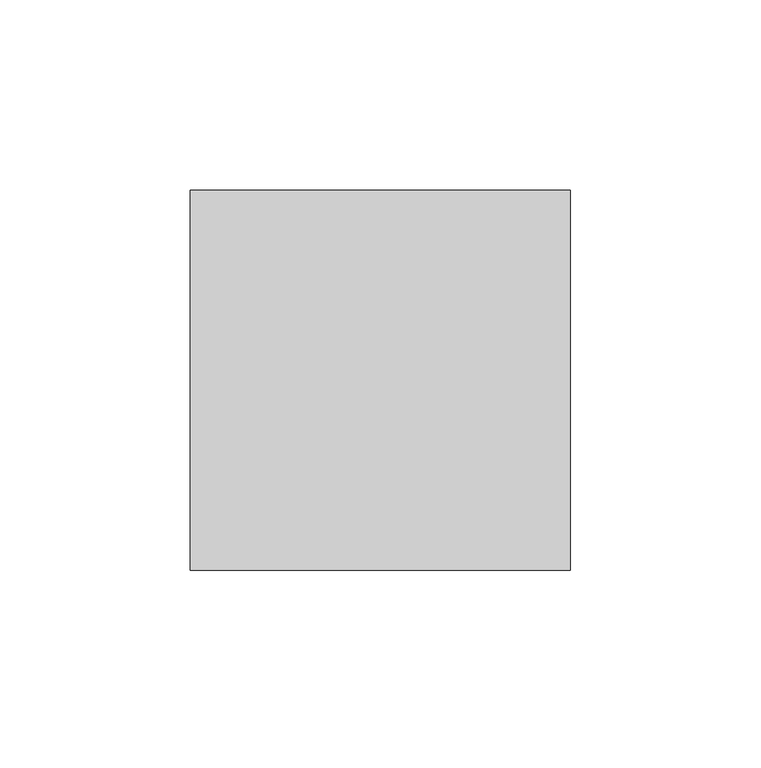
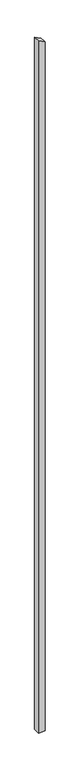
"""IFC4 building model written with IfcOpenShell, lengths in millimetres: column geometry, Holzstütze 159656 : Holzstütze 159656."""

import ifcopenshell
import ifcopenshell.guid

model = None  # the IFC model being written
_history = None  # IfcOwnerHistory: only IFC2X3 demands one
_inside = {}  # id of a spatial element -> (the spatial element, [elements in it])
_under = {}  # id of a project, library or spatial element -> (it, [spatial elements below it])
_declared = {}  # id of a project -> (the project, [libraries it declares])
_typed = {}  # id of a type object -> (the type object, [elements of that type])
_made_of = {}  # id of a material, layer set ... -> (it, [elements and type objects made of it])


def new_model(schema):
    """Start an empty IFC model of exactly this schema.

    Asked for "IFC4X3", IfcOpenShell would pick the latest addendum, in which some entities
    have other attributes; the version numbers below select the first issue.
    IFC2X3 requires an IfcOwnerHistory on every rooted entity: one is made here for all.
    """
    global model, _history
    if schema == "IFC4X3":
        model = ifcopenshell.file(schema_version=(4, 3, 0, 0))
    else:
        model = ifcopenshell.file(schema=schema)
    _inside.clear()
    _under.clear()
    _declared.clear()
    _typed.clear()
    _made_of.clear()
    _history = None
    if model.schema == "IFC2X3":
        org = make("IfcOrganization", Name="unknown")
        user = make(
            "IfcPersonAndOrganization",
            ThePerson=make("IfcPerson", FamilyName="unknown"),
            TheOrganization=org,
        )
        app = make(
            "IfcApplication",
            ApplicationDeveloper=org,
            Version="unknown",
            ApplicationFullName="unknown",
            ApplicationIdentifier="unknown",
        )
        _history = make(
            "IfcOwnerHistory",
            OwningUser=user,
            OwningApplication=app,
            ChangeAction="ADDED",
            CreationDate=0,
        )
    return model


def make(cls, **values):
    """One entity of the class cls with the attributes given. An attribute that is None is left unset."""
    return model.create_entity(
        cls, **{name: value for name, value in values.items() if value is not None}
    )


def rooted(cls, **values):
    """An entity with a GlobalId (a new one), such as an element, a storey or a relation."""
    return make(cls, GlobalId=ifcopenshell.guid.new(), OwnerHistory=_history, **values)


def si_unit(unit_type, name, prefix=None):
    """IfcSIUnit, for example si_unit("LENGTHUNIT", "METRE", prefix="MILLI")."""
    return make("IfcSIUnit", UnitType=unit_type, Prefix=prefix, Name=name)


def assignment(units):
    """IfcUnitAssignment: the units of a project."""
    return None if units is None else make("IfcUnitAssignment", Units=units)


def point(xyz):
    """IfcCartesianPoint."""
    return None if xyz is None else make("IfcCartesianPoint", Coordinates=xyz)


def direction(xyz):
    """IfcDirection."""
    return None if xyz is None else make("IfcDirection", DirectionRatios=xyz)


def frame(location, z_axis=None, x_axis=None):
    """IfcAxis2Placement3D, a coordinate frame: its origin and axes. An axis left out is left unset."""
    return make(
        "IfcAxis2Placement3D",
        Location=point(location),
        Axis=direction(z_axis),
        RefDirection=direction(x_axis),
    )


def origin():
    """The frame at (0, 0, 0) with its axes left unset."""
    return frame((0.0, 0.0, 0.0))


def place(relative_to, where):
    """IfcLocalPlacement: puts the frame where relative to a parent placement (None: the world)."""
    return make(
        "IfcLocalPlacement", PlacementRelTo=relative_to, RelativePlacement=where
    )


def context(
    kind, dimensions, precision=None, world=None, true_north=None, identifier=None
):
    """IfcGeometricRepresentationContext, for example the 3D "Model" context."""
    return make(
        "IfcGeometricRepresentationContext",
        ContextIdentifier=identifier,
        ContextType=kind,
        CoordinateSpaceDimension=dimensions,
        Precision=precision,
        WorldCoordinateSystem=world,
        TrueNorth=true_north,
    )


def project(units=None, contexts=None):
    """IfcProject with its units and contexts."""
    return rooted(
        "IfcProject",
        Name="project",
        RepresentationContexts=contexts,
        UnitsInContext=assignment(units),
    )


def spatial(cls, under=None, at=None, **own):
    """A site, building, storey or space (cls), placed at a placement, below another one or the project."""
    s = rooted(cls, ObjectPlacement=at, **own)
    if under is not None:
        _under.setdefault(under.id(), (under, []))[1].append(s)
    return s


def polyline(points):
    """IfcPolyline through the points."""
    return make("IfcPolyline", Points=[point(p) for p in points])


def outline(outer, holes=None, kind="AREA"):
    """IfcArbitraryClosedProfileDef: a profile drawn as a closed curve; with holes, ...WithVoids."""
    if holes is None:
        return make("IfcArbitraryClosedProfileDef", ProfileType=kind, OuterCurve=outer)
    return make(
        "IfcArbitraryProfileDefWithVoids",
        ProfileType=kind,
        OuterCurve=outer,
        InnerCurves=holes,
    )


def extrude(swept, where, along, depth):
    """IfcExtrudedAreaSolid: the profile swept, set in the frame where, extruded along a direction by depth."""
    return make(
        "IfcExtrudedAreaSolid",
        SweptArea=swept,
        Position=where,
        ExtrudedDirection=direction(along),
        Depth=depth,
    )


def shape(context_of_items, identifier, shape_type, items):
    """IfcShapeRepresentation: the items that make up one representation, for example the "Body"."""
    return make(
        "IfcShapeRepresentation",
        ContextOfItems=context_of_items,
        RepresentationIdentifier=identifier,
        RepresentationType=shape_type,
        Items=items,
    )


def source(mapping_origin, context_of_items, identifier, shape_type, items):
    """IfcRepresentationMap: a shape defined once, which mapped items show again and again."""
    return make(
        "IfcRepresentationMap",
        MappingOrigin=mapping_origin,
        MappedRepresentation=shape(context_of_items, identifier, shape_type, items),
    )


def transform(
    local_origin,
    x_axis=None,
    y_axis=None,
    z_axis=None,
    scale=None,
    scale2=None,
    scale3=None,
    uniform=True,
):
    """IfcCartesianTransformationOperator3D, or its non-uniform kind. x_axis, y_axis, z_axis: its Axis1, 2, 3."""
    if uniform:
        return make(
            "IfcCartesianTransformationOperator3D",
            Axis1=direction(x_axis),
            Axis2=direction(y_axis),
            LocalOrigin=point(local_origin),
            Scale=scale,
            Axis3=direction(z_axis),
        )
    return make(
        "IfcCartesianTransformationOperator3DnonUniform",
        Axis1=direction(x_axis),
        Axis2=direction(y_axis),
        LocalOrigin=point(local_origin),
        Scale=scale,
        Axis3=direction(z_axis),
        Scale2=scale2,
        Scale3=scale3,
    )


def mapped(mapping_source, mapping_target):
    """IfcMappedItem: shows the shape of a source again, moved by a transform."""
    return make(
        "IfcMappedItem", MappingSource=mapping_source, MappingTarget=mapping_target
    )


def made_of(thing, what):
    """Note that an element or type object is made of a material, layer set ...; save() writes the relation."""
    if what is not None:
        _made_of.setdefault(what.id(), (what, []))[1].append(thing)
    return thing


def element(
    cls,
    number,
    at=None,
    inside=None,
    cuts=None,
    type_object=None,
    material=None,
    context=None,
    identifier="Body",
    shape_type=None,
    held_by="IfcProductDefinitionShape",
    body=None,
    shapes=None,
    **own,
):
    """One element of the class cls, such as IfcWall. Its Tag is "e" and its number.

    at: its placement. inside: the storey or other place that contains it. cuts: it is an
    opening in that element (IfcRelVoidsElement). A single representation is given by context,
    identifier, shape_type and body (its items); several are given by shapes. held_by: the class
    of the entity that holds the representations. save() writes the other relations.
    """
    e = rooted(cls, Tag="e%d" % number, ObjectPlacement=at, **own)
    if body is not None:
        shapes = [shape(context, identifier, shape_type, body)]
    if shapes is not None:
        e.Representation = make(held_by, Representations=shapes)
    if inside is not None:
        _inside.setdefault(inside.id(), (inside, []))[1].append(e)
    if cuts is not None:
        rooted(
            "IfcRelVoidsElement", RelatingBuildingElement=cuts, RelatedOpeningElement=e
        )
    if type_object is not None:
        _typed.setdefault(type_object.id(), (type_object, []))[1].append(e)
    return made_of(e, material)


def aggregate(whole, parts):
    """IfcRelAggregates: a whole, such as a stair, and the parts it consists of."""
    return rooted("IfcRelAggregates", RelatingObject=whole, RelatedObjects=parts)


def save(model, path):
    """Write the relations noted so far, then the file.

    IfcRelAggregates (storeys below a building ...), IfcRelContainedInSpatialStructure (elements
    in a storey), IfcRelDefinesByType, IfcRelAssociatesMaterial and IfcRelDeclares: one each for
    every whole, place, type object, material and project.
    """
    for whole, parts in _under.values():
        aggregate(whole, parts)
    for where, things in _inside.values():
        rooted(
            "IfcRelContainedInSpatialStructure",
            RelatedElements=things,
            RelatingStructure=where,
        )
    for kind, things in _typed.values():
        rooted("IfcRelDefinesByType", RelatedObjects=things, RelatingType=kind)
    for what, things in _made_of.values():
        rooted("IfcRelAssociatesMaterial", RelatedObjects=things, RelatingMaterial=what)
    for by, libraries in _declared.values():
        rooted("IfcRelDeclares", RelatingContext=by, RelatedDefinitions=libraries)
    model.write(path)


def column_c1a18ea8(model_context):
    return source(origin(), model_context, "Body", "SweptSolid", [
        extrude(outline(polyline([(-500.0, 165867.7593015), (-500.0, 165967.7593015), (10590.0588201, 165967.7593015), (10641.011365, 165867.7593015), (-500.0, 165867.7593015)])), frame((0.0, 26981.9343946, 0.0), z_axis=(0.0, 1.0, 0.0), x_axis=(0.0, 0.0, 1.0)), (0.0, 0.0, 1.0), 100.0),
    ])


if __name__ == "__main__":
    model = new_model("IFC4")
    model_context = context("Model", 3, world=origin())
    ifc_project = project(units=[si_unit("LENGTHUNIT", "METRE", prefix="MILLI")], contexts=[model_context])
    site = spatial("IfcSite", under=ifc_project)
    building = spatial("IfcBuilding", under=site)
    placement = place(None, origin())
    column_shape = column_c1a18ea8(model_context)
    element("IfcColumn", 1, ObjectType="Holzstütze 159656 : Holzstütze 159656", at=placement, inside=building, context=model_context, shape_type="MappedRepresentation", body=[
        mapped(column_shape, transform((0.0, 0.0, 0.0), x_axis=(1.0, 0.0, 0.0), y_axis=(0.0, 1.0, 0.0), z_axis=(0.0, 0.0, 1.0))),
    ])
    save(model, "model.ifc")

# Revit data of these elements
# Type "Holzstütze 159656 : Holzstütze 159656"
#   Abrechnungsart = "m"
#   Allright_Bauteil_ID = "0152St 0000143519"
#   Bezeichnung = "Holzstütze"
#   Codetext = "ST-HOLZ\\"
#   Gewerk = "Zimmer- und Holzbauarbeiten"
#   Material = "Holz"
#   Objektname = "Stütze"
#   NameOverride = "Holzstütze"
#   Reference = "Holzstütze"
#   Status = "NEW"
#   ThermalTransmittance = 0.0000 BTU/(h·ft²·°F)
#   Roll = 0.00°
#   Slope = 0.00°
#   2D Interaktion = yes
#   IsExternal = yes
#   LoadBearing = yes
# Element 1 (IfcColumn, "Holzstütze 159656 : Holzstütze 159656")
#   Materials on its faces: "holzschalung"
# Materials
#   "holzschalung": class "Unassigned", colour RGB 128 128 128, transparency 0
